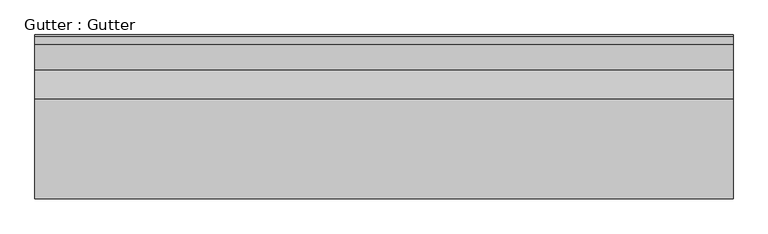
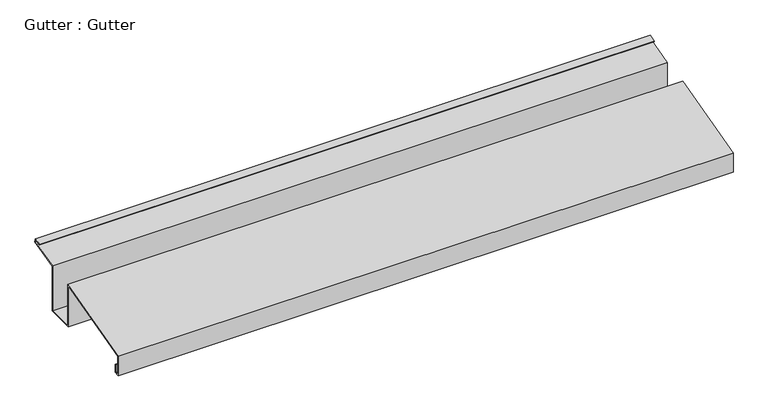
"""IFC4 building model written with IfcOpenShell, lengths in millimetres: proxy geometry, Gutter : Gutter."""

from ifc_helpers import new_model, si_unit, frame, origin, place, context, project, spatial, polyline, outline, extrude, source, transform, mapped, element, save


def gutter_gutter_4af62660(model_context):
    return source(origin(), model_context, "Body", "SweptSolid", [
        extrude(outline(polyline([(-5603.5887201, 42700.9879789), (-5603.5887201, 42673.0479789), (-5621.3687201, 42673.0479789), (-5621.3687201, 42739.4471419), (-5336.549844, 42814.8665333), (-5336.549844, 42672.141563), (-5251.515638, 42672.141563), (-5251.515638, 42825.9077053), (-5154.761123, 42850.915099), (-5156.7473957, 42858.6000602), (-5177.4967906, 42853.237124), (-5178.0926724, 42855.5426123), (-5155.0377891, 42861.5014303), (-5151.8597529, 42849.2054925), (-5249.134388, 42824.0636673), (-5249.134388, 42669.601563), (-5339.089844, 42669.601563), (-5339.089844, 42811.566406), (-5618.8287201, 42737.492187), (-5618.8287201, 42675.5879789), (-5606.1287201, 42675.5879789), (-5606.1287201, 42700.9879789), (-5603.5887201, 42700.9879789)])), frame((12382.7678845, 0.0, 0.0), z_axis=(1.0, 0.0, 0.0), x_axis=(0.0, 1.0, 0.0)), (0.0, 0.0, 1.0), 2000.25),
    ])


if __name__ == "__main__":
    model = new_model("IFC4")
    model_context = context("Model", 3, world=origin())
    ifc_project = project(units=[si_unit("LENGTHUNIT", "METRE", prefix="MILLI")], contexts=[model_context])
    site = spatial("IfcSite", under=ifc_project)
    building = spatial("IfcBuilding", under=site)
    placement = place(None, origin())
    gutter_gutter_shape = gutter_gutter_4af62660(model_context)
    element("IfcBuildingElementProxy", 1, Name="Gutter : Gutter", ObjectType="Gutter : Gutter", at=placement, inside=building, context=model_context, shape_type="MappedRepresentation", body=[
        mapped(gutter_gutter_shape, transform((0.0, 0.0, 0.0), x_axis=(1.0, 0.0, 0.0), y_axis=(0.0, 1.0, 0.0), z_axis=(0.0, 0.0, 1.0))),
    ])
    save(model, "model.ifc")

# Revit data of these elements
# Type "Gutter : Gutter"
#   NameOverride = "Gutter"
# Element 1 (IfcBuildingElementProxy, "Gutter : Gutter")
#   Materials on its faces: "CONT. SEAMLESS 16 GA COPPER BRAKE METAL GUTTER"
# Materials
#   "CONT. SEAMLESS 16 GA COPPER BRAKE METAL GUTTER": class "Unassigned", colour RGB 128 128 128, transparency 0
